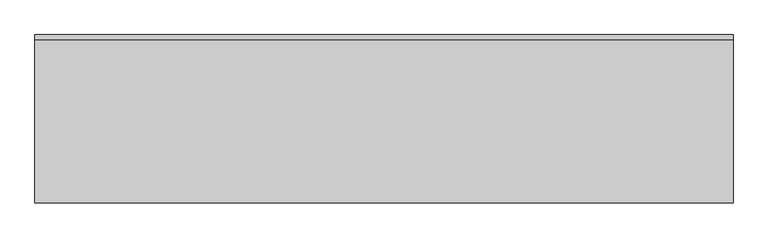
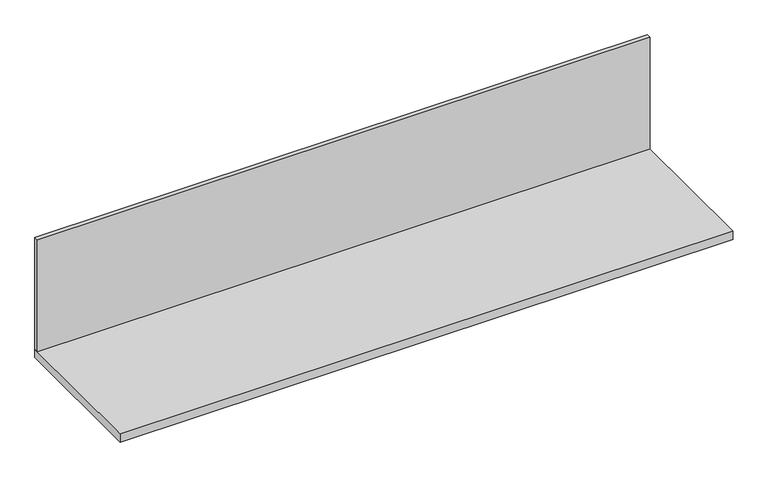
"""IFC4 building model written with IfcOpenShell, lengths in millimetres: furniture geometry, Countertop with Full Backsplash-NON-COLLECTUS : -."""

from ifc_helpers import new_model, si_unit, frame, origin, origin_with_axes, place, context, project, spatial, polyline, outline, extrude, source, transform, mapped, element, save


def furniture_2b8d4a82(model_context):
    return source(origin(), model_context, "Body", "SweptSolid", [
        extrude(outline(polyline([(-1200.4622951, 0.0), (1435.9224321, 0.0), (1435.9224321, -19.05), (-1200.4622951, -19.05), (-1200.4622951, 0.0)])), frame((0.0, 0.0, 38.1), z_axis=(0.0, 0.0, 1.0), x_axis=(1.0, 0.0, 0.0)), (0.0, 0.0, 1.0), 507.5989086),
        extrude(outline(polyline([(1435.9224321, 0.0), (1435.9224321, -634.99873), (-1200.4622951, -634.99873), (-1200.4622951, 0.0), (1435.9224321, 0.0)])), origin_with_axes(), (0.0, 0.0, 1.0), 38.1),
    ])


if __name__ == "__main__":
    model = new_model("IFC4")
    model_context = context("Model", 3, world=origin())
    ifc_project = project(units=[si_unit("LENGTHUNIT", "METRE", prefix="MILLI")], contexts=[model_context])
    site = spatial("IfcSite", under=ifc_project)
    building = spatial("IfcBuilding", under=site)
    placement = place(None, origin())
    furniture_shape = furniture_2b8d4a82(model_context)
    element("IfcFurniture", 1, ObjectType="Countertop with Full Backsplash-NON-COLLECTUS : -", at=placement, inside=building, context=model_context, shape_type="MappedRepresentation", body=[
        mapped(furniture_shape, transform((0.0, 0.0, 0.0), x_axis=(1.0, 0.0, 0.0), y_axis=(0.0, 1.0, 0.0), z_axis=(0.0, 0.0, 1.0))),
    ])
    save(model, "model.ifc")

# Revit data of these elements
# Type "Countertop with Full Backsplash-NON-COLLECTUS : -"
#   External ID [instance default] = ""
#   Width Reporting [instance default] = 1524 mm
#   Width [instance default] = 1524 mm
#   Height Reporting [instance default] = 546.1 mm
#   Depth Reporting [instance default] = 635 mm
#   Depth [instance default] = 635 mm
#   Height [instance default] = 546.1 mm
#   Backsplash = yes
#   Material = White
#   Default Elevation = 0
#   Assembly Code = ""
# Element 1 (IfcFurniture, "Countertop with Full Backsplash-NON-COLLECTUS : -")
#   Width Reporting = 2636.385 mm
#   Width = 2636.385 mm
#   Height Reporting = 545.699 mm
#   Depth Reporting = 634.999 mm
#   Depth = 634.999 mm
#   Height = 545.699 mm
#   Materials on its faces: "White"
# Materials
#   "White": class "Generic", colour RGB 255 255 255, transparency 0, Cost = 0
